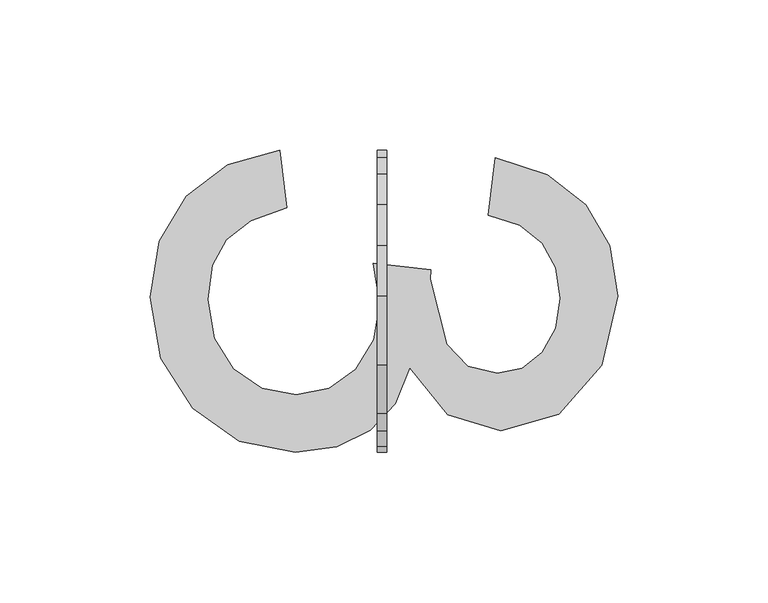
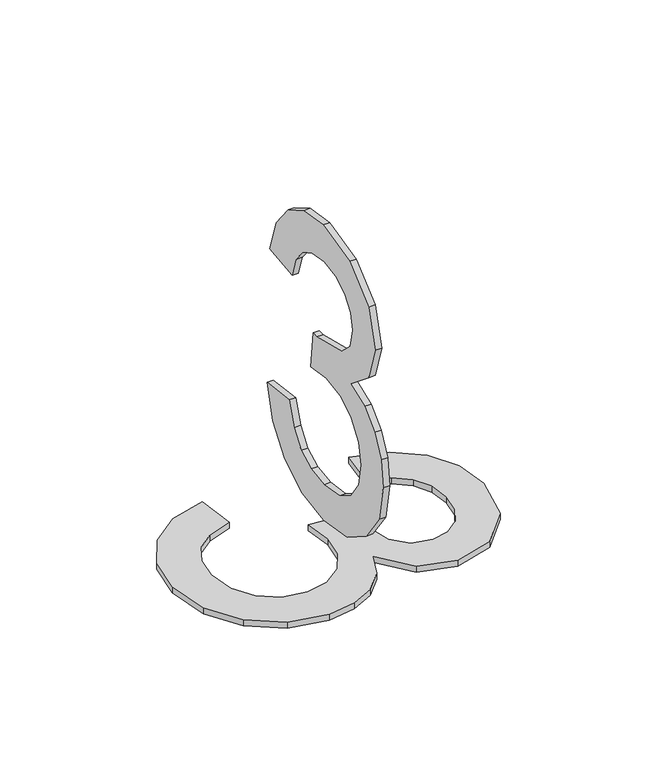
"""IFC4 building model written with IfcOpenShell, lengths in millimetres: proxy geometry, Grid Number2_FedEx : Grid Number2_FedEx."""

import ifcopenshell
import ifcopenshell.guid

model = None  # the IFC model being written
_history = None  # IfcOwnerHistory: only IFC2X3 demands one
_inside = {}  # id of a spatial element -> (the spatial element, [elements in it])
_under = {}  # id of a project, library or spatial element -> (it, [spatial elements below it])
_declared = {}  # id of a project -> (the project, [libraries it declares])
_typed = {}  # id of a type object -> (the type object, [elements of that type])
_made_of = {}  # id of a material, layer set ... -> (it, [elements and type objects made of it])


def new_model(schema):
    """Start an empty IFC model of exactly this schema.

    Asked for "IFC4X3", IfcOpenShell would pick the latest addendum, in which some entities
    have other attributes; the version numbers below select the first issue.
    IFC2X3 requires an IfcOwnerHistory on every rooted entity: one is made here for all.
    """
    global model, _history
    if schema == "IFC4X3":
        model = ifcopenshell.file(schema_version=(4, 3, 0, 0))
    else:
        model = ifcopenshell.file(schema=schema)
    _inside.clear()
    _under.clear()
    _declared.clear()
    _typed.clear()
    _made_of.clear()
    _history = None
    if model.schema == "IFC2X3":
        org = make("IfcOrganization", Name="unknown")
        user = make(
            "IfcPersonAndOrganization",
            ThePerson=make("IfcPerson", FamilyName="unknown"),
            TheOrganization=org,
        )
        app = make(
            "IfcApplication",
            ApplicationDeveloper=org,
            Version="unknown",
            ApplicationFullName="unknown",
            ApplicationIdentifier="unknown",
        )
        _history = make(
            "IfcOwnerHistory",
            OwningUser=user,
            OwningApplication=app,
            ChangeAction="ADDED",
            CreationDate=0,
        )
    return model


def make(cls, **values):
    """One entity of the class cls with the attributes given. An attribute that is None is left unset."""
    return model.create_entity(
        cls, **{name: value for name, value in values.items() if value is not None}
    )


def rooted(cls, **values):
    """An entity with a GlobalId (a new one), such as an element, a storey or a relation."""
    return make(cls, GlobalId=ifcopenshell.guid.new(), OwnerHistory=_history, **values)


def si_unit(unit_type, name, prefix=None):
    """IfcSIUnit, for example si_unit("LENGTHUNIT", "METRE", prefix="MILLI")."""
    return make("IfcSIUnit", UnitType=unit_type, Prefix=prefix, Name=name)


def assignment(units):
    """IfcUnitAssignment: the units of a project."""
    return None if units is None else make("IfcUnitAssignment", Units=units)


def point(xyz):
    """IfcCartesianPoint."""
    return None if xyz is None else make("IfcCartesianPoint", Coordinates=xyz)


def direction(xyz):
    """IfcDirection."""
    return None if xyz is None else make("IfcDirection", DirectionRatios=xyz)


def frame(location, z_axis=None, x_axis=None):
    """IfcAxis2Placement3D, a coordinate frame: its origin and axes. An axis left out is left unset."""
    return make(
        "IfcAxis2Placement3D",
        Location=point(location),
        Axis=direction(z_axis),
        RefDirection=direction(x_axis),
    )


def origin():
    """The frame at (0, 0, 0) with its axes left unset."""
    return frame((0.0, 0.0, 0.0))


def origin_with_axes():
    """The frame at (0, 0, 0) with the z axis (0, 0, 1) and the x axis (1, 0, 0) written out."""
    return frame((0.0, 0.0, 0.0), z_axis=(0.0, 0.0, 1.0), x_axis=(1.0, 0.0, 0.0))


def place(relative_to, where):
    """IfcLocalPlacement: puts the frame where relative to a parent placement (None: the world)."""
    return make(
        "IfcLocalPlacement", PlacementRelTo=relative_to, RelativePlacement=where
    )


def context(
    kind, dimensions, precision=None, world=None, true_north=None, identifier=None
):
    """IfcGeometricRepresentationContext, for example the 3D "Model" context."""
    return make(
        "IfcGeometricRepresentationContext",
        ContextIdentifier=identifier,
        ContextType=kind,
        CoordinateSpaceDimension=dimensions,
        Precision=precision,
        WorldCoordinateSystem=world,
        TrueNorth=true_north,
    )


def project(units=None, contexts=None):
    """IfcProject with its units and contexts."""
    return rooted(
        "IfcProject",
        Name="project",
        RepresentationContexts=contexts,
        UnitsInContext=assignment(units),
    )


def spatial(cls, under=None, at=None, **own):
    """A site, building, storey or space (cls), placed at a placement, below another one or the project."""
    s = rooted(cls, ObjectPlacement=at, **own)
    if under is not None:
        _under.setdefault(under.id(), (under, []))[1].append(s)
    return s


def polyline(points):
    """IfcPolyline through the points."""
    return make("IfcPolyline", Points=[point(p) for p in points])


def outline(outer, holes=None, kind="AREA"):
    """IfcArbitraryClosedProfileDef: a profile drawn as a closed curve; with holes, ...WithVoids."""
    if holes is None:
        return make("IfcArbitraryClosedProfileDef", ProfileType=kind, OuterCurve=outer)
    return make(
        "IfcArbitraryProfileDefWithVoids",
        ProfileType=kind,
        OuterCurve=outer,
        InnerCurves=holes,
    )


def extrude(swept, where, along, depth):
    """IfcExtrudedAreaSolid: the profile swept, set in the frame where, extruded along a direction by depth."""
    return make(
        "IfcExtrudedAreaSolid",
        SweptArea=swept,
        Position=where,
        ExtrudedDirection=direction(along),
        Depth=depth,
    )


def shape(context_of_items, identifier, shape_type, items):
    """IfcShapeRepresentation: the items that make up one representation, for example the "Body"."""
    return make(
        "IfcShapeRepresentation",
        ContextOfItems=context_of_items,
        RepresentationIdentifier=identifier,
        RepresentationType=shape_type,
        Items=items,
    )


def source(mapping_origin, context_of_items, identifier, shape_type, items):
    """IfcRepresentationMap: a shape defined once, which mapped items show again and again."""
    return make(
        "IfcRepresentationMap",
        MappingOrigin=mapping_origin,
        MappedRepresentation=shape(context_of_items, identifier, shape_type, items),
    )


def transform(
    local_origin,
    x_axis=None,
    y_axis=None,
    z_axis=None,
    scale=None,
    scale2=None,
    scale3=None,
    uniform=True,
):
    """IfcCartesianTransformationOperator3D, or its non-uniform kind. x_axis, y_axis, z_axis: its Axis1, 2, 3."""
    if uniform:
        return make(
            "IfcCartesianTransformationOperator3D",
            Axis1=direction(x_axis),
            Axis2=direction(y_axis),
            LocalOrigin=point(local_origin),
            Scale=scale,
            Axis3=direction(z_axis),
        )
    return make(
        "IfcCartesianTransformationOperator3DnonUniform",
        Axis1=direction(x_axis),
        Axis2=direction(y_axis),
        LocalOrigin=point(local_origin),
        Scale=scale,
        Axis3=direction(z_axis),
        Scale2=scale2,
        Scale3=scale3,
    )


def mapped(mapping_source, mapping_target):
    """IfcMappedItem: shows the shape of a source again, moved by a transform."""
    return make(
        "IfcMappedItem", MappingSource=mapping_source, MappingTarget=mapping_target
    )


def made_of(thing, what):
    """Note that an element or type object is made of a material, layer set ...; save() writes the relation."""
    if what is not None:
        _made_of.setdefault(what.id(), (what, []))[1].append(thing)
    return thing


def element(
    cls,
    number,
    at=None,
    inside=None,
    cuts=None,
    type_object=None,
    material=None,
    context=None,
    identifier="Body",
    shape_type=None,
    held_by="IfcProductDefinitionShape",
    body=None,
    shapes=None,
    **own,
):
    """One element of the class cls, such as IfcWall. Its Tag is "e" and its number.

    at: its placement. inside: the storey or other place that contains it. cuts: it is an
    opening in that element (IfcRelVoidsElement). A single representation is given by context,
    identifier, shape_type and body (its items); several are given by shapes. held_by: the class
    of the entity that holds the representations. save() writes the other relations.
    """
    e = rooted(cls, Tag="e%d" % number, ObjectPlacement=at, **own)
    if body is not None:
        shapes = [shape(context, identifier, shape_type, body)]
    if shapes is not None:
        e.Representation = make(held_by, Representations=shapes)
    if inside is not None:
        _inside.setdefault(inside.id(), (inside, []))[1].append(e)
    if cuts is not None:
        rooted(
            "IfcRelVoidsElement", RelatingBuildingElement=cuts, RelatedOpeningElement=e
        )
    if type_object is not None:
        _typed.setdefault(type_object.id(), (type_object, []))[1].append(e)
    return made_of(e, material)


def aggregate(whole, parts):
    """IfcRelAggregates: a whole, such as a stair, and the parts it consists of."""
    return rooted("IfcRelAggregates", RelatingObject=whole, RelatedObjects=parts)


def save(model, path):
    """Write the relations noted so far, then the file.

    IfcRelAggregates (storeys below a building ...), IfcRelContainedInSpatialStructure (elements
    in a storey), IfcRelDefinesByType, IfcRelAssociatesMaterial and IfcRelDeclares: one each for
    every whole, place, type object, material and project.
    """
    for whole, parts in _under.values():
        aggregate(whole, parts)
    for where, things in _inside.values():
        rooted(
            "IfcRelContainedInSpatialStructure",
            RelatedElements=things,
            RelatingStructure=where,
        )
    for kind, things in _typed.values():
        rooted("IfcRelDefinesByType", RelatedObjects=things, RelatingType=kind)
    for what, things in _made_of.values():
        rooted("IfcRelAssociatesMaterial", RelatedObjects=things, RelatingMaterial=what)
    for by, libraries in _declared.values():
        rooted("IfcRelDeclares", RelatingContext=by, RelatedDefinitions=libraries)
    model.write(path)


def entourage_147b0573(model_context):
    return source(origin(), model_context, "Body", "SweptSolid", [
        extrude(outline(polyline([(-143.6079567, 271.5590522), (-141.2158408, 252.4221251), (-153.2418296, 248.1378082), (-161.3619418, 241.8631761), (-165.9873221, 233.2898701), (-167.5291155, 222.1095316), (-165.4079815, 208.990271), (-159.0445795, 198.8611553), (-149.5508696, 192.3856229), (-138.0388119, 190.2271121), (-127.1107669, 192.3669345), (-118.2477906, 198.7864017), (-112.3749592, 208.5043725), (-110.4173488, 220.5397056), (-112.5104502, 233.9579806), (-93.3735231, 231.8275024), (-93.597784, 228.7626039), (-88.1033928, 207.0466769), (-81.1326176, 199.814264), (-71.2090743, 197.4034597), (-62.9441271, 199.1508256), (-56.2396617, 204.3929233), (-51.7964933, 212.3915608), (-50.3154372, 222.4085461), (-51.8105096, 232.4442198), (-56.2957269, 240.6484297), (-63.771089, 246.6380636), (-74.236596, 250.0300092), (-71.8444801, 269.1669363), (-54.6604914, 263.5323821), (-41.8309011, 253.5060526), (-33.8416078, 239.7887631), (-31.1785101, 223.0813287), (-36.429952, 200.0011481), (-50.7826473, 183.8543658), (-70.08777, 178.2665326), (-87.7296247, 183.5740398), (-100.4003635, 199.2723003), (-105.2406605, 187.2930324), (-113.4822473, 178.4160399), (-124.6766021, 172.9216487), (-138.3752032, 171.090185), (-157.0262317, 174.7531124), (-172.6123618, 185.7418948), (-183.1526224, 202.3278545), (-186.6660426, 222.7823142), (-183.6665536, 241.2838355), (-174.6680864, 256.3466902), (-160.9040758, 266.8215414), (-143.6079567, 271.5590522)])), origin_with_axes(), (0.0, 0.0, 1.0), 3.175),
        extrude(outline(polyline([(271.5590522, 54.9042454), (266.8215414, 37.6081262), (256.3466902, 23.8441157), (241.2838355, 14.8456485), (222.7823142, 11.8461594), (202.3278545, 15.3595796), (185.7418948, 25.8998402), (174.7531124, 41.4859703), (171.090185, 60.1369989), (172.9216487, 73.8356), (178.4160399, 85.0299548), (187.2930324, 93.2715416), (199.2723003, 98.1118385), (183.5740398, 110.7825774), (178.2665326, 128.424432), (183.8543658, 147.7295548), (200.0011481, 162.0822501), (223.0813287, 167.333692), (239.7887631, 164.6705942), (253.5060526, 156.6813009), (263.5323821, 143.8517106), (269.1669363, 126.6677219), (250.0300092, 124.275606), (246.6380636, 134.741113), (240.6484297, 142.2164752), (232.4442198, 146.7016925), (222.4085461, 148.1967649), (212.3915608, 146.7157088), (204.3929233, 142.2725404), (199.1508256, 135.568075), (197.4034597, 127.3031277), (199.814264, 117.3795845), (207.0466769, 110.4088093), (228.7626039, 104.9144181), (231.8275024, 105.138679), (233.9579806, 86.0017519), (220.5397056, 88.0948533), (208.5043725, 86.1372428), (198.7864017, 80.2644114), (192.3669345, 71.4014352), (190.2271121, 60.4733902), (192.3856229, 48.9613325), (198.8611553, 39.4676225), (208.990271, 33.1042205), (222.1095316, 30.9830865), (233.2898701, 32.5248799), (241.8631761, 37.1502603), (248.1378082, 45.2703724), (252.4221251, 57.2963612), (271.5590522, 54.9042454)])), frame((-111.2489267, 0.0, 0.0), z_axis=(1.0, 0.0, 0.0), x_axis=(0.0, 1.0, 0.0)), (0.0, 0.0, 1.0), 3.175),
    ])


if __name__ == "__main__":
    model = new_model("IFC4")
    model_context = context("Model", 3, world=origin())
    ifc_project = project(units=[si_unit("LENGTHUNIT", "METRE", prefix="MILLI")], contexts=[model_context])
    site = spatial("IfcSite", under=ifc_project)
    building = spatial("IfcBuilding", under=site)
    placement = place(None, origin())
    entourage_shape = entourage_147b0573(model_context)
    element("IfcBuildingElementProxy", 1, Name="Grid Number2_FedEx : Grid Number2_FedEx", ObjectType="Grid Number2_FedEx : Grid Number2_FedEx", at=placement, inside=building, context=model_context, shape_type="MappedRepresentation", body=[
        mapped(entourage_shape, transform((0.0, 0.0, 0.0), x_axis=(1.0, 0.0, 0.0), y_axis=(0.0, 1.0, 0.0), z_axis=(0.0, 0.0, 1.0))),
    ])
    save(model, "model.ifc")

# Revit data of these elements
# Type "Grid Number2_FedEx : Grid Number2_FedEx"
#   Grid [instance default] = "S"
#   Label Width [instance default] = 1' - 0"
#   Half Box Width2 [instance default] = 0' - 6.13846"
#   Half Box Width [instance default] = 0' - 6"
#   Robust [instance default] = yes
#   Height = 0
#   Assembly Code = ""
# Element 1 (IfcBuildingElementProxy, "Grid Number2_FedEx : Grid Number2_FedEx")
#   Grid = "3"
#   Robust = no
#   Materials on its faces: "Letter"
# Materials
#   "Letter": class "Unassigned", colour RGB 178 187 30, transparency 0, Comments = "Rendering appearance not upgraded "
